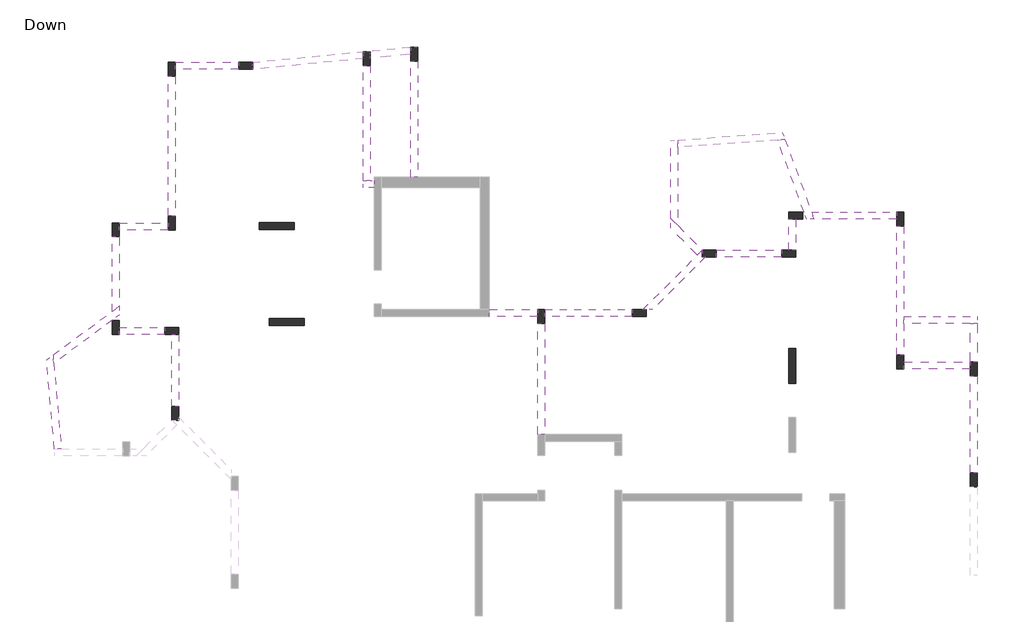
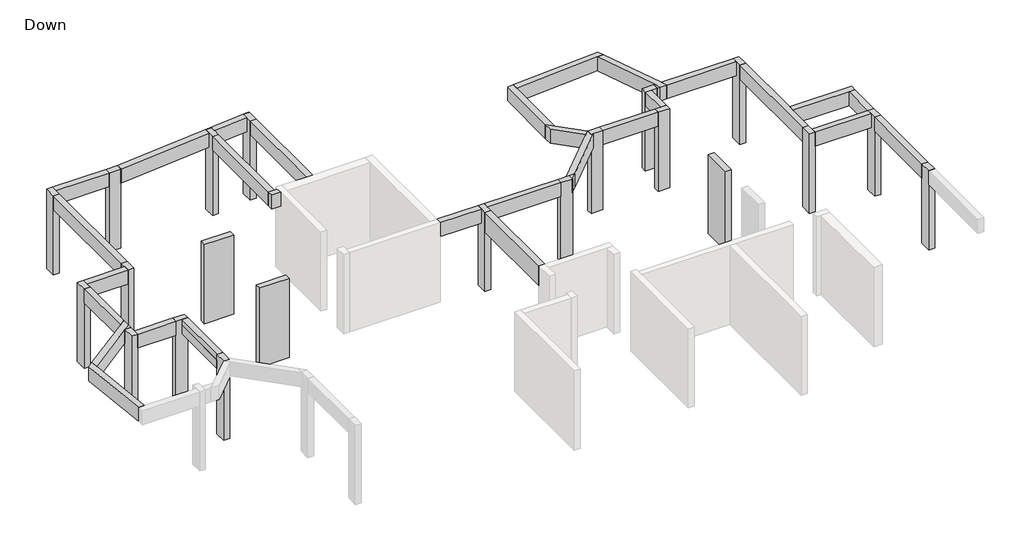
# One storey, part 3 of 3: 28 beams, 21 columns.
"""IFC4 building model written with IfcOpenShell, lengths in millimetres."""

from ifc_helpers import new_model, si_unit, frame, origin, origin_with_axes, place, context, project, spatial, polyline, outline, extrude, faceted_brep, element, save

model = new_model("IFC4")

# Units and contexts
model_context = context("Model", 3, world=origin())
ifc_project = project(units=[si_unit("LENGTHUNIT", "METRE", prefix="MILLI")], contexts=[model_context])

# Site, building, storey
site = spatial("IfcSite", under=ifc_project)
building = spatial("IfcBuilding", under=site)
storey = spatial("IfcBuildingStorey", under=building, Name="Down", Elevation=0.0)

# Beams
placement = place(None, origin())
element("IfcBeam", 1, ObjectType="Concrete Rectengular Beam : 20/50", at=placement, inside=storey, context=model_context, shape_type="Brep", body=[
    faceted_brep([(-18653.293728, -891.3531176, 2850.0), (-18452.5305511, -891.3531176, 2850.0), (-18667.1860705, 1563.4435406, 2850.0), (-18687.6029963, 1796.9311366, 2850.0), (-18876.1976023, 1657.7715773, 2850.0), (-18687.6029963, 1796.9311366, 2350.0), (-18452.5305511, -891.3531176, 2650.0), (-18452.5305511, -891.3531176, 2350.0), (-18667.1860705, 1563.4435406, 2350.0), (-18653.293728, -891.3531176, 2350.0), (-18876.1976023, 1657.7715773, 2350.0)], [[[0, 1, 2, 3, 4]], [[5, 3, 2, 1, 6, 7, 8]], [[7, 9, 10, 5, 8]], [[9, 0, 4, 10]], [[1, 0, 9, 7, 6]], [[4, 3, 5, 10]]]),
])
element("IfcBeam", 2, ObjectType="Concrete Rectengular Beam : 20/50", at=placement, inside=storey, context=model_context, shape_type="Brep", body=[
    faceted_brep([(-18687.6029963, 1796.9311366, 2850.0), (-18667.1860705, 1563.4435406, 2850.0), (-16994.2441564, 2797.8683443, 2850.0), (-16794.2441564, 2945.4436777, 2850.0), (-16794.2441564, 3193.9964468, 2850.0), (-16994.2441564, 3046.4211134, 2850.0), (-16794.2441564, 2945.4436777, 2350.0), (-18667.1860705, 1563.4435406, 2650.0), (-18667.1860705, 1563.4435406, 2350.0), (-16994.2441564, 2797.8683443, 2350.0), (-18687.6029963, 1796.9311366, 2350.0), (-16994.2441564, 3046.4211134, 2350.0), (-16794.2441564, 3193.9964468, 2350.0)], [[[0, 1, 2, 3, 4, 5]], [[6, 3, 2, 1, 7, 8, 9]], [[8, 10, 11, 12, 6, 9]], [[10, 0, 5, 4, 12, 11]], [[1, 0, 10, 8, 7]], [[4, 3, 6, 12]]]),
])
element("IfcBeam", 3, ObjectType="Concrete Rectengular Beam : 20/50", at=placement, inside=storey, context=model_context, shape_type="Brep", body=[
    faceted_brep([(-15089.2187138, 316.4585788, 2850.0), (-15089.2187138, 2386.9126556, 2850.0), (-15284.2187138, 2386.9126556, 2850.0), (-15284.2187138, 316.4585788, 2850.0), (-15089.2187138, 316.4585788, 2650.0), (-15089.2187138, 316.4585788, 2350.0), (-15089.2187138, 2386.9126556, 2350.0), (-15089.2187138, 2386.9126556, 2650.0), (-15289.2187138, 2386.9126556, 2350.0), (-15289.2187138, 316.4585788, 2350.0), (-15289.2187138, 316.4585788, 2650.0), (-15289.2187138, 2386.9126556, 2650.0), (-15284.2187138, 2386.9126556, 2650.0), (-15284.2187138, 316.4585788, 2650.0)], [[[0, 1, 2, 3]], [[1, 0, 4, 5, 6, 7]], [[8, 6, 5, 9]], [[8, 9, 10, 11]], [[6, 8, 11, 12, 2, 1, 7]], [[9, 5, 4, 0, 3, 13, 10]], [[13, 12, 11, 10]], [[12, 13, 3, 2]]]),
])
element("IfcBeam", 4, ObjectType="Concrete Rectengular Beam : 20/50", at=placement, inside=storey, context=model_context, shape_type="Brep", body=[
    faceted_brep([(-16794.2441564, 2586.9126556, 2850.0), (-16794.2441564, 2386.9126556, 2850.0), (-15489.2187138, 2386.9126556, 2850.0), (-15489.2187138, 2586.9126556, 2850.0), (-15489.2187138, 2586.9126556, 2650.0), (-15489.2187138, 2586.9126556, 2350.0), (-16794.2441564, 2586.9126556, 2350.0), (-16794.2441564, 2586.9126556, 2650.0), (-16794.2441564, 2386.9126556, 2350.0), (-15489.2187138, 2386.9126556, 2350.0), (-16794.2441564, 2386.9126556, 2650.0), (-15489.2187138, 2386.9126556, 2650.0)], [[[0, 1, 2, 3]], [[0, 3, 4, 5, 6, 7]], [[8, 6, 5, 9]], [[2, 1, 10, 8, 9, 11]], [[1, 0, 7, 6, 8, 10]], [[3, 2, 11, 9, 5, 4]]]),
])
element("IfcBeam", 5, ObjectType="Concrete Rectengular Beam : 20/50", at=placement, inside=storey, context=model_context, shape_type="Brep", body=[
    faceted_brep([(-16794.2441564, 5184.8420774, 2850.0), (-16994.2441564, 5184.8420774, 2850.0), (-16994.2441564, 3046.4211134, 2850.0), (-16794.2441564, 3193.9964468, 2850.0), (-16794.2441564, 5184.8420774, 2350.0), (-16794.2441564, 3193.9964468, 2350.0), (-16994.2441564, 5184.8420774, 2350.0), (-16994.2441564, 3046.4211134, 2350.0)], [[[0, 1, 2, 3]], [[4, 0, 3, 5]], [[6, 4, 5, 7]], [[1, 6, 7, 2]], [[1, 0, 4, 6]], [[3, 2, 7, 5]]]),
    faceted_brep([(-16794.2441564, 2786.9126556, 2850.0), (-16994.2441564, 2786.9126556, 2850.0), (-16994.2441564, 2786.9126556, 2650.0), (-16994.2441564, 2786.9126556, 2350.0), (-16794.2441564, 2786.9126556, 2350.0), (-16994.2441564, 2797.8683443, 2850.0), (-16794.2441564, 2945.4436777, 2850.0), (-16794.2441564, 2945.4436777, 2350.0), (-16994.2441564, 2797.8683443, 2350.0), (-16994.2441564, 2797.8683443, 2650.0)], [[[0, 1, 2, 3, 4]], [[5, 6, 7, 8, 9]], [[1, 0, 6, 5]], [[0, 4, 7, 6]], [[4, 3, 8, 7]], [[1, 5, 9, 8, 3, 2]]]),
])
element("IfcBeam", 6, ObjectType="Concrete Rectengular Beam : 20/50", at=placement, inside=storey, context=model_context, shape_type="Brep", body=[
    faceted_brep([(-15386.5645409, 5384.8420774, 2850.0), (-15386.5645409, 5584.8420774, 2850.0), (-16794.2441564, 5584.8420774, 2850.0), (-16794.2441564, 5384.8420774, 2850.0), (-15386.5645409, 5584.8420774, 2350.0), (-16794.2441564, 5584.8420774, 2350.0), (-15386.5645409, 5384.8420774, 2350.0), (-16794.2441564, 5384.8420774, 2350.0), (-16794.2441564, 5384.8420774, 2650.0), (-15386.5645409, 5384.8420774, 2650.0)], [[[0, 1, 2, 3]], [[1, 4, 5, 2]], [[4, 6, 7, 5]], [[0, 3, 8, 7, 6, 9]], [[1, 0, 9, 6, 4]], [[3, 2, 5, 7, 8]]]),
])
element("IfcBeam", 7, ObjectType="Concrete Rectengular Beam : 20/50", at=placement, inside=storey, context=model_context, shape_type="Brep", body=[
    faceted_brep([(-15186.5645409, 9788.9617999, 2850.0), (-15386.5645409, 9788.9617999, 2850.0), (-15386.5645409, 5784.8420774, 2850.0), (-15186.5645409, 5784.8420774, 2850.0), (-15186.5645409, 5784.8420774, 2650.0), (-15186.5645409, 5784.8420774, 2350.0), (-15186.5645409, 9788.9617999, 2350.0), (-15186.5645409, 9788.9617999, 2650.0), (-15386.5645409, 9788.9617999, 2350.0), (-15386.5645409, 5784.8420774, 2350.0)], [[[0, 1, 2, 3]], [[0, 3, 4, 5, 6, 7]], [[8, 6, 5, 9]], [[1, 8, 9, 2]], [[1, 0, 7, 6, 8]], [[3, 2, 9, 5, 4]]]),
])
element("IfcBeam", 8, ObjectType="Concrete Rectengular Beam : 20/50", at=placement, inside=storey, context=model_context, shape_type="Brep", body=[
    faceted_brep([(-15186.5645409, 10188.9617999, 2850.0), (-15186.5645409, 9988.9617999, 2850.0), (-13373.5990213, 9988.9617999, 2850.0), (-13373.5990213, 10188.9617999, 2850.0), (-15186.5645409, 9988.9617999, 2650.0), (-15186.5645409, 9988.9617999, 2350.0), (-13373.5990213, 9988.9617999, 2350.0), (-13373.5990213, 9988.9617999, 2650.0), (-15186.5645409, 10188.9617999, 2350.0), (-13373.5990213, 10188.9617999, 2350.0)], [[[0, 1, 2, 3]], [[2, 1, 4, 5, 6, 7]], [[5, 8, 9, 6]], [[8, 0, 3, 9]], [[0, 8, 5, 4, 1]], [[3, 2, 7, 6, 9]]]),
    faceted_brep([(-12973.5990213, 10088.9617999, 2850.0), (-12968.8298625, 9988.9617999, 2850.0), (-12968.8298625, 9988.9617999, 2650.0), (-12968.8298625, 9988.9617999, 2350.0), (-12973.5990213, 10088.9617999, 2350.0), (-12973.5990213, 9988.9617999, 2850.0), (-12973.5990213, 9988.9617999, 2350.0), (-12973.5990213, 9988.9617999, 2650.0)], [[[0, 1, 2, 3, 4]], [[5, 0, 4, 6, 7]], [[1, 0, 5]], [[1, 5, 7, 6, 3, 2]], [[4, 3, 6]]]),
])
element("IfcBeam", 9, ObjectType="Concrete Rectengular Beam : 20/50", at=placement, inside=storey, context=model_context, shape_type="Brep", body=[
    faceted_brep([(-8256.1274624, 10640.4109367, 2850.0), (-12978.3681802, 10188.9617999, 2850.0), (-12973.5990213, 10188.9617999, 2850.0), (-12973.5990213, 10088.9617999, 2850.0), (-12968.8298625, 9988.9617999, 2850.0), (-9797.9493855, 10292.099937, 2850.0), (-9797.9493855, 10422.4041492, 2850.0), (-9797.9493855, 10488.7487212, 2850.0), (-9597.9493855, 10488.7487212, 2850.0), (-9597.9493855, 10422.4041492, 2850.0), (-9597.9493855, 10311.2200609, 2850.0), (-8437.0941181, 10422.1985433, 2850.0), (-8437.0941181, 10622.4041492, 2850.0), (-8254.4060024, 10622.4041492, 2850.0), (-9597.9493855, 10311.2200609, 2650.0), (-9597.9493855, 10311.2200609, 2350.0), (-8437.0941181, 10422.1985433, 2350.0), (-8437.0941181, 10422.1985433, 2650.0), (-12978.3681802, 10188.9617999, 2350.0), (-8256.1274624, 10640.4109367, 2350.0), (-8254.4060024, 10622.4041492, 2350.0), (-8437.0941181, 10622.4041492, 2350.0), (-9597.9493855, 10422.4041492, 2350.0), (-9597.9493855, 10488.7487212, 2350.0), (-9797.9493855, 10488.7487212, 2350.0), (-9797.9493855, 10422.4041492, 2350.0), (-9797.9493855, 10292.099937, 2350.0), (-12968.8298625, 9988.9617999, 2350.0), (-12973.5990213, 10088.9617999, 2350.0), (-12973.5990213, 10188.9617999, 2350.0), (-12968.8298625, 9988.9617999, 2650.0), (-9797.9493855, 10292.099937, 2650.0)], [[[0, 1, 2, 3, 4, 5, 6, 7, 8, 9, 10, 11, 12, 13]], [[11, 10, 14, 15, 16, 17]], [[18, 19, 20, 21, 16, 15, 22, 23, 24, 25, 26, 27, 28, 29]], [[1, 0, 19, 18]], [[4, 3, 28, 27, 30]], [[19, 0, 13, 20]], [[29, 2, 1, 18]], [[2, 29, 28, 3]], [[21, 12, 11, 17, 16]], [[12, 21, 20, 13]], [[24, 7, 6, 5, 31, 26, 25]], [[7, 24, 23, 8]], [[8, 23, 22, 15, 14, 10, 9]], [[5, 4, 30, 27, 26, 31]]]),
])
element("IfcBeam", 10, ObjectType="Concrete Rectengular Beam : 20/50", at=placement, inside=storey, context=model_context, shape_type="Brep", body=[
    faceted_brep([(-8237.0941181, 10222.4041492, 2850.0), (-8437.0941181, 10222.4041492, 2850.0), (-8437.0941181, 6897.8899275, 2850.0), (-8237.0941181, 6897.8899275, 2850.0), (-8437.0941181, 10222.4041492, 2350.0), (-8437.0941181, 6897.8899275, 2350.0), (-8437.0941181, 6897.8899275, 2650.0), (-8237.0941181, 10222.4041492, 2350.0), (-8237.0941181, 6897.8899275, 2350.0)], [[[0, 1, 2, 3]], [[1, 4, 5, 6, 2]], [[4, 7, 8, 5]], [[7, 0, 3, 8]], [[1, 0, 7, 4]], [[3, 2, 6, 5, 8]]]),
])
element("IfcBeam", 11, ObjectType="Concrete Rectengular Beam : 20/50", at=placement, inside=storey, context=model_context, shape_type="Brep", body=[
    faceted_brep([(-9490.6856227, 6598.9542002, 2850.0), (-9490.6856227, 6798.9542002, 2850.0), (-9597.9493855, 6798.9542002, 2850.0), (-9797.9493855, 6798.9542002, 2850.0), (-9797.9493855, 6598.9542002, 2850.0), (-9490.6856227, 6798.9542002, 2650.0), (-9490.6856227, 6798.9542002, 2350.0), (-9597.9493855, 6798.9542002, 2350.0), (-9797.9493855, 6798.9542002, 2350.0), (-9797.9493855, 6798.9542002, 2650.0), (-9490.6856227, 6598.9542002, 2350.0), (-9797.9493855, 6598.9542002, 2350.0), (-9797.9493855, 6598.9542002, 2650.0), (-9490.6856227, 6598.9542002, 2650.0)], [[[0, 1, 2, 3, 4]], [[1, 5, 6, 7, 8, 9, 3, 2]], [[6, 10, 11, 8, 7]], [[0, 4, 12, 11, 10, 13]], [[1, 0, 13, 10, 6, 5]], [[4, 3, 9, 8, 11, 12]]]),
])
element("IfcBeam", 12, ObjectType="Concrete Rectengular Beam : 20/50", at=placement, inside=storey, context=model_context, shape_type="Brep", body=[
    faceted_brep([(-9597.9493855, 10088.7487212, 2850.0), (-9797.9493855, 10088.7487212, 2850.0), (-9797.9493855, 6798.9542002, 2850.0), (-9597.9493855, 6798.9542002, 2850.0), (-9597.9493855, 10088.7487212, 2350.0), (-9597.9493855, 6798.9542002, 2650.0), (-9597.9493855, 6798.9542002, 2350.0), (-9797.9493855, 10088.7487212, 2350.0), (-9797.9493855, 6798.9542002, 2350.0), (-9797.9493855, 10088.7487212, 2650.0), (-9797.9493855, 6798.9542002, 2650.0)], [[[0, 1, 2, 3]], [[4, 0, 3, 5, 6]], [[7, 4, 6, 8]], [[2, 1, 9, 7, 8, 10]], [[1, 0, 4, 7, 9]], [[3, 2, 10, 8, 6, 5]]]),
])
element("IfcBeam", 13, ObjectType="Concrete Rectengular Beam : 20/50", at=placement, inside=storey, context=model_context, shape_type="Brep", body=[
    faceted_brep([(-4797.6379386, 2895.9323955, 2850.0), (-4797.6379386, 3095.9323955, 2850.0), (-6200.1625371, 3095.9323955, 2850.0), (-6200.1625371, 2895.9323955, 2850.0), (-4797.6379386, 3095.9323955, 2350.0), (-6200.1625371, 3095.9323955, 2350.0), (-4797.6379386, 2895.9323955, 2350.0), (-6200.1625371, 2895.9323955, 2350.0), (-6200.1625371, 2895.9323955, 2650.0), (-4797.6379386, 2895.9323955, 2650.0)], [[[0, 1, 2, 3]], [[1, 4, 5, 2]], [[4, 6, 7, 5]], [[0, 3, 8, 7, 6, 9]], [[1, 0, 9, 6, 4]], [[3, 2, 5, 7, 8]]]),
])
element("IfcBeam", 14, ObjectType="Concrete Rectengular Beam : 20/50", at=placement, inside=storey, context=model_context, shape_type="Brep", body=[
    faceted_brep([(-2099.1198792, 2895.9323955, 2850.0), (-2099.1198792, 3095.9323955, 2850.0), (-4597.6379386, 3095.9323955, 2850.0), (-4597.6379386, 2895.9323955, 2850.0), (-4597.6379386, 2895.9323955, 2650.0), (-4597.6379386, 2895.9323955, 2350.0), (-2099.1198792, 2895.9323955, 2350.0), (-2099.1198792, 2895.9323955, 2650.0), (-2099.1198792, 3095.9323955, 2350.0), (-4597.6379386, 3095.9323955, 2350.0)], [[[0, 1, 2, 3]], [[0, 3, 4, 5, 6, 7]], [[8, 6, 5, 9]], [[1, 8, 9, 2]], [[1, 0, 7, 6, 8]], [[3, 2, 9, 5, 4]]]),
    faceted_brep([(-1512.3548664, 3095.9323955, 2850.0), (-1699.1198792, 2909.1673916, 2850.0), (-1699.1198792, 2909.1673916, 2650.0), (-1699.1198792, 2909.1673916, 2350.0), (-1512.3548664, 3095.9323955, 2350.0), (-1512.3548664, 3095.9323955, 2650.0), (-1699.1198792, 3095.9323955, 2850.0), (-1699.1198792, 3095.9323955, 2350.0)], [[[0, 1, 2, 3, 4, 5]], [[1, 6, 7, 3, 2]], [[0, 6, 1]], [[7, 4, 3]], [[6, 0, 5, 4, 7]]]),
])
element("IfcBeam", 15, ObjectType="Concrete Rectengular Beam : 20/50", at=placement, inside=storey, context=model_context, shape_type="Brep", body=[
    faceted_brep([(-9.6892647, 4598.5979252, 2850.0), (-89.77599, 4598.5979252, 2850.0), (-89.77599, 4798.5979252, 2850.0), (-83.949, 4798.5979252, 2850.0), (-88.2404871, 4802.8894122, 2850.0), (-229.6618467, 4661.4680594, 2850.0), (-1795.1975857, 3095.9323955, 2850.0), (-1699.1198792, 3095.9323955, 2850.0), (-1512.3548664, 3095.9323955, 2850.0), (-1512.3548664, 3095.9323955, 2650.0), (-1512.3548664, 3095.9323955, 2350.0), (-9.6892647, 4598.5979252, 2350.0), (-9.6892647, 4598.5979252, 2650.0), (-89.77599, 4598.5979252, 2350.0), (-1699.1198792, 3095.9323955, 2350.0), (-1795.1975857, 3095.9323955, 2350.0), (-229.6618467, 4661.4680594, 2350.0), (-88.2404871, 4802.8894122, 2350.0), (-83.949, 4798.5979252, 2350.0), (-89.77599, 4798.5979252, 2350.0), (-88.2404871, 4802.8894122, 2650.0), (-83.949, 4798.5979252, 2650.0)], [[[0, 1, 2, 3, 4, 5, 6, 7, 8]], [[0, 8, 9, 10, 11, 12]], [[13, 11, 10, 14, 15, 16, 17, 18, 19]], [[15, 6, 5, 4, 20, 17, 16]], [[13, 1, 0, 12, 11]], [[1, 13, 19, 2]], [[8, 7, 6, 15, 14, 10, 9]], [[4, 3, 21, 18, 17, 20]], [[2, 19, 18, 21, 3]]]),
])
element("IfcBeam", 16, ObjectType="Concrete Rectengular Beam : 20/50", at=placement, inside=storey, context=model_context, shape_type="Brep", body=[
    faceted_brep([(-229.6618467, 4661.4680594, 2850.0), (-88.2404871, 4802.8894122, 2850.0), (-799.5327681, 5514.1816932, 2850.0), (-999.5327681, 5714.1816932, 2850.0), (-999.5327681, 5431.3389807, 2850.0), (-999.5327681, 5714.1816932, 2350.0), (-88.2404871, 4802.8894122, 2650.0), (-88.2404871, 4802.8894122, 2350.0), (-799.5327681, 5514.1816932, 2350.0), (-229.6618467, 4661.4680594, 2350.0), (-999.5327681, 5431.3389807, 2350.0)], [[[0, 1, 2, 3, 4]], [[5, 3, 2, 1, 6, 7, 8]], [[7, 9, 10, 5, 8]], [[9, 0, 4, 10]], [[1, 0, 9, 7, 6]], [[4, 3, 5, 10]]]),
])
element("IfcBeam", 17, ObjectType="Concrete Rectengular Beam : 20/50", at=placement, inside=storey, context=model_context, shape_type="Brep", body=[
    faceted_brep([(-999.5327681, 5714.1816932, 2850.0), (-799.5327681, 5514.1816932, 2850.0), (-799.5327681, 7759.5088284, 2850.0), (-799.5327681, 7959.997208, 2850.0), (-999.5327681, 7946.0118456, 2850.0), (-799.5327681, 5514.1816932, 2650.0), (-799.5327681, 5514.1816932, 2350.0), (-799.5327681, 7759.5088284, 2350.0), (-799.5327681, 7959.997208, 2350.0), (-999.5327681, 5714.1816932, 2350.0), (-999.5327681, 7946.0118456, 2350.0)], [[[0, 1, 2, 3, 4]], [[1, 5, 6, 7, 8, 3, 2]], [[6, 9, 10, 8, 7]], [[9, 0, 4, 10]], [[1, 0, 9, 6, 5]], [[4, 3, 8, 10]]]),
])
element("IfcBeam", 18, ObjectType="Concrete Rectengular Beam : 20/50", at=placement, inside=storey, context=model_context, shape_type="Brep", body=[
    faceted_brep([(-799.5327681, 7959.997208, 2850.0), (-799.5327681, 7759.5088284, 2850.0), (2065.6791891, 7959.8639661, 2850.0), (2273.4365693, 7974.3917773, 2850.0), (2201.5390264, 8169.852591, 2850.0), (2273.4365693, 7974.3917773, 2350.0), (-799.5327681, 7759.5088284, 2650.0), (-799.5327681, 7759.5088284, 2350.0), (2065.6791891, 7959.8639661, 2350.0), (-799.5327681, 7959.997208, 2350.0), (2201.5390264, 8169.852591, 2350.0)], [[[0, 1, 2, 3, 4]], [[5, 3, 2, 1, 6, 7, 8]], [[7, 9, 10, 5, 8]], [[9, 0, 4, 10]], [[1, 0, 9, 7, 6]], [[4, 3, 5, 10]]]),
])
element("IfcBeam", 19, ObjectType="Concrete Rectengular Beam : 20/50", at=placement, inside=storey, context=model_context, shape_type="Brep", body=[
    faceted_brep([(2273.4365693, 7974.3917773, 2850.0), (2065.6791891, 7959.8639661, 2850.0), (2826.2618446, 5892.1423364, 2850.0), (2899.8290642, 5692.1423364, 2850.0), (3112.9302979, 5692.1423364, 2850.0), (3039.3630783, 5892.1423364, 2850.0), (2899.8290642, 5692.1423364, 2350.0), (2065.6791891, 7959.8639661, 2650.0), (2065.6791891, 7959.8639661, 2350.0), (2826.2618446, 5892.1423364, 2350.0), (2273.4365693, 7974.3917773, 2350.0), (3039.3630783, 5892.1423364, 2350.0), (3112.9302979, 5692.1423364, 2350.0)], [[[0, 1, 2, 3, 4, 5]], [[6, 3, 2, 1, 7, 8, 9]], [[8, 10, 11, 12, 6, 9]], [[10, 0, 5, 4, 12, 11]], [[1, 0, 10, 8, 7]], [[4, 3, 6, 12]]]),
])
element("IfcBeam", 20, ObjectType="Concrete Rectengular Beam : 20/50", at=placement, inside=storey, context=model_context, shape_type="Brep", body=[
    faceted_brep([(2189.104476, 4598.5979252, 2850.0), (2189.104476, 4798.5979252, 2850.0), (310.22401, 4798.5979252, 2850.0), (310.22401, 4598.5979252, 2850.0), (310.22401, 4598.5979252, 2650.0), (310.22401, 4598.5979252, 2350.0), (2189.104476, 4598.5979252, 2350.0), (2189.104476, 4598.5979252, 2650.0), (2189.104476, 4798.5979252, 2350.0), (310.22401, 4798.5979252, 2350.0)], [[[0, 1, 2, 3]], [[0, 3, 4, 5, 6, 7]], [[8, 6, 5, 9]], [[1, 8, 9, 2]], [[1, 0, 7, 6, 8]], [[3, 2, 9, 5, 4]]]),
])
element("IfcBeam", 21, ObjectType="Concrete Rectengular Beam : 20/50", at=placement, inside=storey, context=model_context, shape_type="Brep", body=[
    faceted_brep([(2589.104476, 5692.1423364, 2850.0), (2389.104476, 5692.1423364, 2850.0), (2389.104476, 4798.5979252, 2850.0), (2589.104476, 4798.5979252, 2850.0), (2389.104476, 5692.1423364, 2650.0), (2389.104476, 5692.1423364, 2350.0), (2389.104476, 4798.5979252, 2350.0), (2389.104476, 4798.5979252, 2650.0), (2589.104476, 5692.1423364, 2350.0), (2589.104476, 4798.5979252, 2350.0), (2589.104476, 4798.5979252, 2650.0), (2589.104476, 5692.1423364, 2650.0)], [[[0, 1, 2, 3]], [[2, 1, 4, 5, 6, 7]], [[5, 8, 9, 6]], [[0, 3, 10, 9, 8, 11]], [[1, 0, 11, 8, 5, 4]], [[3, 2, 7, 6, 9, 10]]]),
])
element("IfcBeam", 22, ObjectType="Concrete Rectengular Beam : 20/50", at=placement, inside=storey, context=model_context, shape_type="Brep", body=[
    faceted_brep([(5484.9828456, 5692.1423364, 2850.0), (5484.9828456, 5892.1423364, 2850.0), (3039.3630783, 5892.1423364, 2850.0), (3112.9302979, 5692.1423364, 2850.0), (5484.9828456, 5692.1423364, 2350.0), (5484.9828456, 5692.1423364, 2650.0), (3112.9302979, 5692.1423364, 2350.0), (5484.9828456, 5892.1423364, 2350.0), (3039.3630783, 5892.1423364, 2350.0)], [[[0, 1, 2, 3]], [[4, 5, 0, 3, 6]], [[7, 4, 6, 8]], [[1, 7, 8, 2]], [[1, 0, 5, 4, 7]], [[3, 2, 8, 6]]]),
    faceted_brep([(2789.104476, 5692.1423364, 2850.0), (2789.104476, 5892.1423364, 2850.0), (2789.104476, 5892.1423364, 2650.0), (2789.104476, 5892.1423364, 2350.0), (2789.104476, 5692.1423364, 2350.0), (2826.2618446, 5892.1423364, 2850.0), (2899.8290642, 5692.1423364, 2850.0), (2899.8290642, 5692.1423364, 2350.0), (2826.2618446, 5892.1423364, 2350.0), (2826.2618446, 5892.1423364, 2650.0)], [[[0, 1, 2, 3, 4]], [[5, 6, 7, 8, 9]], [[1, 0, 6, 5]], [[0, 4, 7, 6]], [[4, 3, 8, 7]], [[1, 5, 9, 8, 3, 2]]]),
])
element("IfcBeam", 23, ObjectType="Concrete Rectengular Beam : 20/50", at=placement, inside=storey, context=model_context, shape_type="Brep", body=[
    faceted_brep([(5484.9828456, 1795.5159248, 2850.0), (5684.9828456, 1795.5159248, 2850.0), (5684.9828456, 2705.1624293, 2850.0), (5684.9828456, 2905.1624293, 2850.0), (5684.9828456, 5494.9383888, 2850.0), (5484.9828456, 5494.9383888, 2850.0), (5484.9828456, 5494.9383888, 2650.0), (5484.9828456, 5494.9383888, 2350.0), (5484.9828456, 1795.5159248, 2350.0), (5484.9828456, 1795.5159248, 2650.0), (5684.9828456, 1795.5159248, 2350.0), (5684.9828456, 5494.9383888, 2350.0), (5684.9828456, 2905.1624293, 2350.0), (5684.9828456, 2705.1624293, 2350.0)], [[[0, 1, 2, 3, 4, 5]], [[0, 5, 6, 7, 8, 9]], [[10, 8, 7, 11, 12, 13]], [[1, 10, 13, 12, 11, 4, 3, 2]], [[1, 0, 9, 8, 10]], [[5, 4, 11, 7, 6]]]),
])
element("IfcBeam", 24, ObjectType="Concrete Rectengular Beam : 20/50", at=placement, inside=storey, context=model_context, shape_type="Brep", body=[
    faceted_brep([(5684.9828456, 2905.1624293, 2850.0), (5684.9828456, 2705.1624293, 2850.0), (7591.3944084, 2705.1624293, 2850.0), (7791.3944084, 2705.1624293, 2850.0), (7791.3944084, 2905.1624293, 2850.0), (5684.9828456, 2705.1624293, 2650.0), (5684.9828456, 2705.1624293, 2350.0), (7591.3944084, 2705.1624293, 2350.0), (7791.3944084, 2705.1624293, 2350.0), (5684.9828456, 2905.1624293, 2350.0), (7791.3944084, 2905.1624293, 2350.0)], [[[0, 1, 2, 3, 4]], [[1, 5, 6, 7, 8, 3, 2]], [[6, 9, 10, 8, 7]], [[9, 0, 4, 10]], [[1, 0, 9, 6, 5]], [[4, 3, 8, 10]]]),
])
element("IfcBeam", 25, ObjectType="Concrete Rectengular Beam : 20/50", at=placement, inside=storey, context=model_context, shape_type="Brep", body=[
    faceted_brep([(7591.3944084, 1595.5159248, 2850.0), (7791.3944084, 1595.5159248, 2850.0), (7791.3944084, 2705.1624293, 2850.0), (7591.3944084, 2705.1624293, 2850.0), (7591.3944084, 1595.5159248, 2350.0), (7591.3944084, 1595.5159248, 2650.0), (7591.3944084, 2705.1624293, 2650.0), (7591.3944084, 2705.1624293, 2350.0), (7791.3944084, 1595.5159248, 2350.0), (7791.3944084, 2705.1624293, 2350.0)], [[[0, 1, 2, 3]], [[4, 5, 0, 3, 6, 7]], [[8, 4, 7, 9]], [[1, 8, 9, 2]], [[1, 0, 5, 4, 8]], [[3, 2, 9, 7, 6]]]),
])
element("IfcBeam", 26, ObjectType="Concrete Rectengular Beam : 20/50", at=placement, inside=storey, context=model_context, shape_type="Brep", body=[
    faceted_brep([(7591.3944084, 1395.5159248, 2850.0), (7591.3944084, 1595.5159248, 2850.0), (5684.9828456, 1595.5159248, 2850.0), (5684.9828456, 1395.5159248, 2850.0), (7591.3944084, 1595.5159248, 2650.0), (7591.3944084, 1595.5159248, 2350.0), (5684.9828456, 1595.5159248, 2350.0), (5684.9828456, 1595.5159248, 2650.0), (7591.3944084, 1395.5159248, 2350.0), (5684.9828456, 1395.5159248, 2350.0), (5684.9828456, 1395.5159248, 2650.0), (7591.3944084, 1395.5159248, 2650.0)], [[[0, 1, 2, 3]], [[1, 4, 5, 6, 7, 2]], [[5, 8, 9, 6]], [[0, 3, 10, 9, 8, 11]], [[1, 0, 11, 8, 5, 4]], [[3, 2, 7, 6, 9, 10]]]),
])
element("IfcBeam", 27, ObjectType="Concrete Rectengular Beam : 20/50", at=placement, inside=storey, context=model_context, shape_type="SweptSolid", body=[
    extrude(outline(polyline([(7791.3944084, -1588.6737606), (7591.3944084, -1588.6737606), (7591.3944084, 1195.5159248), (7791.3944084, 1195.5159248), (7791.3944084, -1588.6737606)])), frame((0.0, 0.0, 2350.0), z_axis=(0.0, 0.0, 1.0), x_axis=(1.0, 0.0, 0.0)), (0.0, 0.0, 1.0), 500.0),
])
element("IfcBeam", 28, ObjectType="Concrete Rectengular Beam : 20/70", at=placement, inside=storey, context=model_context, shape_type="Brep", body=[
    faceted_brep([(-4597.6379386, 2696.2012144, 2850.0), (-4797.6379386, 2696.2012144, 2850.0), (-4797.6379386, -483.2914692, 2850.0), (-4597.6379386, -483.2914692, 2850.0), (-4797.6379386, 2696.2012144, 2650.0), (-4797.6379386, 2696.2012144, 2150.0), (-4797.6379386, -483.2914692, 2150.0), (-4797.6379386, -483.2914692, 2650.0), (-4597.6379386, 2696.2012144, 2150.0), (-4597.6379386, -483.2914692, 2150.0), (-4597.6379386, -483.2914692, 2650.0)], [[[0, 1, 2, 3]], [[2, 1, 4, 5, 6, 7]], [[5, 8, 9, 6]], [[8, 0, 3, 10, 9]], [[1, 0, 8, 5, 4]], [[3, 2, 7, 6, 9, 10]]]),
])

# Columns
element("IfcColumn", 29, ObjectType="Concrete Rectengular Column : 100/20", at=placement, inside=storey, context=model_context, shape_type="Brep", body=[
    faceted_brep([(2387.619868, 1976.5237192, 0.0), (2587.619868, 1976.5237192, 0.0), (2587.619868, 976.5237192, 0.0), (2387.619868, 976.5237192, 0.0), (2387.619868, 1976.5237192, 2850.0), (2587.619868, 1976.5237192, 2850.0), (2587.619868, 1976.5237192, 2650.0), (2387.619868, 1976.5237192, 2650.0), (2587.619868, 976.5237192, 2850.0), (2587.619868, 976.5237192, 2650.0), (2387.619868, 976.5237192, 2850.0), (2387.619868, 976.5237192, 2650.0)], [[[0, 1, 2, 3]], [[4, 5, 6, 1, 0, 7]], [[5, 8, 9, 2, 1, 6]], [[8, 10, 11, 3, 2, 9]], [[10, 4, 7, 0, 3, 11]], [[4, 10, 8, 5]]]),
])
element("IfcColumn", 30, ObjectType="Concrete Rectengular Column : 100/20", at=placement, inside=storey, context=model_context, shape_type="Brep", body=[
    faceted_brep([(-12489.8453542, 2637.5348136, 0.0), (-12489.8453542, 2837.5348136, 0.0), (-11489.8453542, 2837.5348136, 0.0), (-11489.8453542, 2637.5348136, 0.0), (-12489.8453542, 2637.5348136, 2850.0), (-12489.8453542, 2837.5348136, 2850.0), (-12489.8453542, 2837.5348136, 2650.0), (-12489.8453542, 2637.5348136, 2650.0), (-11489.8453542, 2837.5348136, 2850.0), (-11489.8453542, 2837.5348136, 2650.0), (-11489.8453542, 2637.5348136, 2850.0), (-11489.8453542, 2637.5348136, 2650.0)], [[[0, 1, 2, 3]], [[4, 5, 6, 1, 0, 7]], [[5, 8, 9, 2, 1, 6]], [[8, 10, 11, 3, 2, 9]], [[10, 4, 7, 0, 3, 11]], [[4, 10, 8, 5]]]),
])
element("IfcColumn", 31, ObjectType="Concrete Rectengular Column : 100/20", at=placement, inside=storey, context=model_context, shape_type="Brep", body=[
    faceted_brep([(-12783.7609512, 5396.0878026, 0.0), (-12783.7609512, 5596.0878026, 0.0), (-11783.7609512, 5596.0878026, 0.0), (-11783.7609512, 5396.0878026, 0.0), (-12783.7609512, 5396.0878026, 2850.0), (-12783.7609512, 5596.0878026, 2850.0), (-12783.7609512, 5596.0878026, 2650.0), (-12783.7609512, 5396.0878026, 2650.0), (-11783.7609512, 5596.0878026, 2850.0), (-11783.7609512, 5596.0878026, 2650.0), (-11783.7609512, 5396.0878026, 2850.0), (-11783.7609512, 5396.0878026, 2650.0)], [[[0, 1, 2, 3]], [[4, 5, 6, 1, 0, 7]], [[5, 8, 9, 2, 1, 6]], [[8, 10, 11, 3, 2, 9]], [[10, 4, 7, 0, 3, 11]], [[4, 10, 8, 5]]]),
])
element("IfcColumn", 32, ObjectType="Concrete Rectengular Column : 20/40", at=placement, inside=storey, context=model_context, shape_type="Brep", body=[
    faceted_brep([(-15186.5645409, 10188.9617999, 0.0), (-15186.5645409, 9788.9617999, 0.0), (-15386.5645409, 9788.9617999, 0.0), (-15386.5645409, 10188.9617999, 0.0), (-15186.5645409, 10188.9617999, 2850.0), (-15186.5645409, 9988.9617999, 2850.0), (-15186.5645409, 9788.9617999, 2850.0), (-15386.5645409, 9788.9617999, 2850.0), (-15386.5645409, 10188.9617999, 2850.0)], [[[0, 1, 2, 3]], [[4, 5, 6, 1, 0]], [[6, 7, 2, 1]], [[7, 8, 3, 2]], [[8, 4, 0, 3]], [[4, 8, 7, 6, 5]]]),
])
element("IfcColumn", 33, ObjectType="Concrete Rectengular Column : 20/40", at=placement, inside=storey, context=model_context, shape_type="SweptSolid", body=[
    extrude(outline(polyline([(-13373.5990213, 10188.9617999), (-12973.5990213, 10188.9617999), (-12973.5990213, 9988.9617999), (-13373.5990213, 9988.9617999), (-13373.5990213, 10188.9617999)])), origin_with_axes(), (0.0, 0.0, 1.0), 2850.0),
])
element("IfcColumn", 34, ObjectType="Concrete Rectengular Column : 20/40", at=placement, inside=storey, context=model_context, shape_type="Brep", body=[
    faceted_brep([(-9797.9493855, 10088.7487212, 0.0), (-9797.9493855, 10488.7487212, 0.0), (-9597.9493855, 10488.7487212, 0.0), (-9597.9493855, 10088.7487212, 0.0), (-9797.9493855, 10088.7487212, 2850.0), (-9797.9493855, 10292.099937, 2850.0), (-9797.9493855, 10488.7487212, 2850.0), (-9797.9493855, 10488.7487212, 2350.0), (-9597.9493855, 10488.7487212, 2850.0), (-9597.9493855, 10488.7487212, 2350.0), (-9597.9493855, 10311.2200609, 2850.0), (-9597.9493855, 10088.7487212, 2850.0)], [[[0, 1, 2, 3]], [[4, 5, 6, 7, 1, 0]], [[6, 8, 9, 2, 1, 7]], [[8, 10, 11, 3, 2, 9]], [[11, 4, 0, 3]], [[4, 11, 10, 8, 6, 5]]]),
])
element("IfcColumn", 35, ObjectType="Concrete Rectengular Column : 20/40", at=placement, inside=storey, context=model_context, shape_type="Brep", body=[
    faceted_brep([(-8437.0941181, 10222.4041492, 0.0), (-8437.0941181, 10622.4041492, 0.0), (-8237.0941181, 10622.4041492, 0.0), (-8237.0941181, 10222.4041492, 0.0), (-8437.0941181, 10222.4041492, 2850.0), (-8437.0941181, 10422.1985433, 2850.0), (-8437.0941181, 10622.4041492, 2850.0), (-8237.0941181, 10622.4041492, 2850.0), (-8237.0941181, 10222.4041492, 2850.0)], [[[0, 1, 2, 3]], [[4, 5, 6, 1, 0]], [[6, 7, 2, 1]], [[7, 8, 3, 2]], [[8, 4, 0, 3]], [[4, 8, 7, 6, 5]]]),
])
element("IfcColumn", 36, ObjectType="Concrete Rectengular Column : 20/40", at=placement, inside=storey, context=model_context, shape_type="Brep", body=[
    faceted_brep([(-15186.5645409, 5784.8420774, 0.0), (-15186.5645409, 5384.8420774, 0.0), (-15386.5645409, 5384.8420774, 0.0), (-15386.5645409, 5784.8420774, 0.0), (-15186.5645409, 5784.8420774, 2850.0), (-15186.5645409, 5384.8420774, 2850.0), (-15186.5645409, 5384.8420774, 2650.0), (-15386.5645409, 5384.8420774, 2850.0), (-15386.5645409, 5784.8420774, 2850.0)], [[[0, 1, 2, 3]], [[4, 5, 6, 1, 0]], [[5, 7, 2, 1, 6]], [[7, 8, 3, 2]], [[8, 4, 0, 3]], [[4, 8, 7, 5]]]),
])
element("IfcColumn", 37, ObjectType="Concrete Rectengular Column : 20/40", at=placement, inside=storey, context=model_context, shape_type="Brep", body=[
    faceted_brep([(-16794.2441564, 5584.8420774, 0.0), (-16794.2441564, 5184.8420774, 0.0), (-16994.2441564, 5184.8420774, 0.0), (-16994.2441564, 5584.8420774, 0.0), (-16794.2441564, 5584.8420774, 2850.0), (-16794.2441564, 5384.8420774, 2850.0), (-16794.2441564, 5184.8420774, 2850.0), (-16994.2441564, 5184.8420774, 2850.0), (-16994.2441564, 5584.8420774, 2850.0)], [[[0, 1, 2, 3]], [[4, 5, 6, 1, 0]], [[6, 7, 2, 1]], [[7, 8, 3, 2]], [[8, 4, 0, 3]], [[4, 8, 7, 6, 5]]]),
])
element("IfcColumn", 38, ObjectType="Concrete Rectengular Column : 20/40", at=placement, inside=storey, context=model_context, shape_type="Brep", body=[
    faceted_brep([(-16794.2441564, 2786.9126556, 0.0), (-16794.2441564, 2386.9126556, 0.0), (-16994.2441564, 2386.9126556, 0.0), (-16994.2441564, 2786.9126556, 0.0), (-16794.2441564, 2786.9126556, 2850.0), (-16794.2441564, 2586.9126556, 2850.0), (-16794.2441564, 2386.9126556, 2850.0), (-16994.2441564, 2386.9126556, 2850.0), (-16994.2441564, 2386.9126556, 2650.0), (-16994.2441564, 2786.9126556, 2850.0)], [[[0, 1, 2, 3]], [[4, 5, 6, 1, 0]], [[6, 7, 8, 2, 1]], [[7, 9, 3, 2, 8]], [[9, 4, 0, 3]], [[4, 9, 7, 6, 5]]]),
])
element("IfcColumn", 39, ObjectType="Concrete Rectengular Column : 20/40", at=placement, inside=storey, context=model_context, shape_type="Brep", body=[
    faceted_brep([(-15489.2187138, 2586.9126556, 0.0), (-15089.2187138, 2586.9126556, 0.0), (-15089.2187138, 2386.9126556, 0.0), (-15489.2187138, 2386.9126556, 0.0), (-15489.2187138, 2586.9126556, 2850.0), (-15089.2187138, 2586.9126556, 2850.0), (-15089.2187138, 2586.9126556, 2650.0), (-15089.2187138, 2386.9126556, 2850.0), (-15284.2187138, 2386.9126556, 2850.0), (-15489.2187138, 2386.9126556, 2850.0)], [[[0, 1, 2, 3]], [[4, 5, 6, 1, 0]], [[5, 7, 2, 1, 6]], [[7, 8, 9, 3, 2]], [[9, 4, 0, 3]], [[4, 9, 8, 7, 5]]]),
])
element("IfcColumn", 40, ObjectType="Concrete Rectengular Column : 20/40", at=placement, inside=storey, context=model_context, shape_type="Brep", body=[
    faceted_brep([(-15289.2187138, -83.5414212, 0.0), (-15289.2187138, 316.4585788, 0.0), (-15089.2187138, 316.4585788, 0.0), (-15089.2187138, -83.5414212, 0.0), (-15289.2187138, -83.5414212, 2850.0), (-15289.2187138, -73.3367957, 2850.0), (-15289.2187138, 316.4585788, 2850.0), (-15289.2187138, 316.4585788, 2650.0), (-15289.2187138, -83.5414212, 2350.0), (-15284.2187138, 316.4585788, 2850.0), (-15089.2187138, 316.4585788, 2850.0), (-15089.2187138, 11.75673, 2850.0), (-15089.2187138, -83.5414212, 2850.0), (-15273.253528, -83.5414212, 2850.0)], [[[0, 1, 2, 3]], [[4, 5, 6, 7, 1, 0, 8]], [[6, 9, 10, 2, 1, 7]], [[10, 11, 12, 3, 2]], [[12, 13, 4, 8, 0, 3]], [[4, 13, 12, 11, 10, 9, 6, 5]]]),
])
element("IfcColumn", 41, ObjectType="Concrete Rectengular Column : 20/40", at=placement, inside=storey, context=model_context, shape_type="SweptSolid", body=[
    extrude(outline(polyline([(7791.3944084, -1588.6737606), (7791.3944084, -1988.6737606), (7591.3944084, -1988.6737606), (7591.3944084, -1588.6737606), (7791.3944084, -1588.6737606)])), origin_with_axes(), (0.0, 0.0, 1.0), 2850.0),
])
element("IfcColumn", 42, ObjectType="Concrete Rectengular Column : 20/40", at=placement, inside=storey, context=model_context, shape_type="Brep", body=[
    faceted_brep([(7591.3944084, 1195.5159248, 0.0), (7591.3944084, 1595.5159248, 0.0), (7791.3944084, 1595.5159248, 0.0), (7791.3944084, 1195.5159248, 0.0), (7591.3944084, 1195.5159248, 2850.0), (7591.3944084, 1395.5159248, 2850.0), (7591.3944084, 1595.5159248, 2850.0), (7791.3944084, 1595.5159248, 2850.0), (7791.3944084, 1195.5159248, 2850.0)], [[[0, 1, 2, 3]], [[4, 5, 6, 1, 0]], [[6, 7, 2, 1]], [[7, 8, 3, 2]], [[8, 4, 0, 3]], [[4, 8, 7, 6, 5]]]),
])
element("IfcColumn", 43, ObjectType="Concrete Rectengular Column : 20/40", at=placement, inside=storey, context=model_context, shape_type="Brep", body=[
    faceted_brep([(5484.9828456, 1395.5159248, 0.0), (5484.9828456, 1795.5159248, 0.0), (5684.9828456, 1795.5159248, 0.0), (5684.9828456, 1395.5159248, 0.0), (5484.9828456, 1395.5159248, 2850.0), (5484.9828456, 1795.5159248, 2850.0), (5484.9828456, 1395.5159248, 2650.0), (5684.9828456, 1795.5159248, 2850.0), (5684.9828456, 1595.5159248, 2850.0), (5684.9828456, 1395.5159248, 2850.0)], [[[0, 1, 2, 3]], [[4, 5, 1, 0, 6]], [[5, 7, 2, 1]], [[7, 8, 9, 3, 2]], [[9, 4, 6, 0, 3]], [[4, 9, 8, 7, 5]]]),
])
element("IfcColumn", 44, ObjectType="Concrete Rectengular Column : 20/40", at=placement, inside=storey, context=model_context, shape_type="Brep", body=[
    faceted_brep([(5484.9828456, 5494.9383888, 0.0), (5484.9828456, 5894.9383888, 0.0), (5684.9828456, 5894.9383888, 0.0), (5684.9828456, 5494.9383888, 0.0), (5484.9828456, 5494.9383888, 2850.0), (5484.9828456, 5692.1423364, 2850.0), (5484.9828456, 5894.9383888, 2850.0), (5684.9828456, 5894.9383888, 2850.0), (5684.9828456, 5494.9383888, 2850.0)], [[[0, 1, 2, 3]], [[4, 5, 6, 1, 0]], [[6, 7, 2, 1]], [[7, 8, 3, 2]], [[8, 4, 0, 3]], [[4, 8, 7, 6, 5]]]),
])
element("IfcColumn", 45, ObjectType="Concrete Rectengular Column : 20/40", at=placement, inside=storey, context=model_context, shape_type="Brep", body=[
    faceted_brep([(2789.104476, 5692.1423364, 0.0), (2389.104476, 5692.1423364, 0.0), (2389.104476, 5892.1423364, 0.0), (2789.104476, 5892.1423364, 0.0), (2789.104476, 5692.1423364, 2850.0), (2589.104476, 5692.1423364, 2850.0), (2389.104476, 5692.1423364, 2850.0), (2389.104476, 5892.1423364, 2850.0), (2389.104476, 5892.1423364, 2650.0), (2789.104476, 5892.1423364, 2850.0)], [[[0, 1, 2, 3]], [[4, 5, 6, 1, 0]], [[6, 7, 8, 2, 1]], [[7, 9, 3, 2, 8]], [[9, 4, 0, 3]], [[4, 9, 7, 6, 5]]]),
])
element("IfcColumn", 46, ObjectType="Concrete Rectengular Column : 20/40", at=placement, inside=storey, context=model_context, shape_type="Brep", body=[
    faceted_brep([(2589.104476, 4598.5979252, 0.0), (2189.104476, 4598.5979252, 0.0), (2189.104476, 4798.5979252, 0.0), (2589.104476, 4798.5979252, 0.0), (2589.104476, 4598.5979252, 2850.0), (2189.104476, 4598.5979252, 2850.0), (2589.104476, 4598.5979252, 2650.0), (2189.104476, 4798.5979252, 2850.0), (2389.104476, 4798.5979252, 2850.0), (2589.104476, 4798.5979252, 2850.0)], [[[0, 1, 2, 3]], [[4, 5, 1, 0, 6]], [[5, 7, 2, 1]], [[7, 8, 9, 3, 2]], [[9, 4, 6, 0, 3]], [[4, 9, 8, 7, 5]]]),
])
element("IfcColumn", 47, ObjectType="Concrete Rectengular Column : 20/40", at=placement, inside=storey, context=model_context, shape_type="Brep", body=[
    faceted_brep([(310.22401, 4598.5979252, 0.0), (-89.77599, 4598.5979252, 0.0), (-89.77599, 4798.5979252, 0.0), (310.22401, 4798.5979252, 0.0), (310.22401, 4598.5979252, 2850.0), (-9.6893457, 4598.5979252, 2850.0), (-89.77599, 4598.5979252, 2850.0), (-89.77599, 4798.5979252, 2850.0), (-83.949, 4798.5979252, 2850.0), (310.22401, 4798.5979252, 2850.0)], [[[0, 1, 2, 3]], [[4, 5, 6, 1, 0]], [[6, 7, 2, 1]], [[7, 8, 9, 3, 2]], [[9, 4, 0, 3]], [[4, 9, 8, 7, 6, 5]]]),
])
element("IfcColumn", 48, ObjectType="Concrete Rectengular Column : 20/40", at=placement, inside=storey, context=model_context, shape_type="Brep", body=[
    faceted_brep([(-1699.1198792, 2895.9323955, 0.0), (-2099.1198792, 2895.9323955, 0.0), (-2099.1198792, 3095.9323955, 0.0), (-1699.1198792, 3095.9323955, 0.0), (-1699.1198792, 2895.9323955, 2850.0), (-2099.1198792, 2895.9323955, 2850.0), (-1699.1198792, 2895.9323955, 2650.0), (-2099.1198792, 3095.9323955, 2850.0), (-1699.1198792, 3095.9323955, 2850.0), (-1699.1198792, 2909.1673916, 2850.0)], [[[0, 1, 2, 3]], [[4, 5, 1, 0, 6]], [[5, 7, 2, 1]], [[7, 8, 3, 2]], [[8, 9, 4, 6, 0, 3]], [[4, 9, 8, 7, 5]]]),
])
element("IfcColumn", 49, ObjectType="Concrete Rectengular Column : 20/40", at=placement, inside=storey, context=model_context, shape_type="Brep", body=[
    faceted_brep([(-4597.6379386, 3096.2012144, 0.0), (-4597.6379386, 2696.2012144, 0.0), (-4797.6379386, 2696.2012144, 0.0), (-4797.6379386, 3096.2012144, 0.0), (-4597.6379386, 3096.2012144, 2850.0), (-4597.6379386, 2895.9323955, 2850.0), (-4597.6379386, 2696.2012144, 2850.0), (-4797.6379386, 2696.2012144, 2850.0), (-4797.6379386, 2895.9323955, 2850.0), (-4797.6379386, 3096.2012144, 2850.0)], [[[0, 1, 2, 3]], [[4, 5, 6, 1, 0]], [[6, 7, 2, 1]], [[7, 8, 9, 3, 2]], [[9, 4, 0, 3]], [[4, 9, 8, 7, 6, 5]]]),
])

save(model, "model.ifc")

# Revit data of these elements
# Type "Concrete Rectengular Beam : 20/50"
#   Length [instance default] = 152.4 cm
#   b = 20 cm
#   h = 50 cm
#   Structural Material [instance default] = Concrete
#   Assembly Code = ""
# Type "Concrete Rectengular Beam : 20/70"
#   Length [instance default] = 152.4 cm
#   b = 20 cm
#   h = 70 cm
#   Structural Material [instance default] = Concrete
#   Assembly Code = ""
# Type "Concrete Rectengular Column : 100/20"
#   b = 100 cm
#   h = 20 cm
#   Structural Material [instance default] = Concrete
# Type "Concrete Rectengular Column : 20/40"
#   b = 20 cm
#   h = 40 cm
#   Structural Material [instance default] = Concrete
# Element 1 (IfcBeam, "Concrete Rectengular Beam : 20/50")
#   Comments = ""
#   Mark = "B22"
#   SOFiSTiK_AMG_Comments = ""
#   SOFiSTiK_AMG_Scheduled = yes
#   SOFiSTiK_AMG_Adjusted = yes
#   Structural Material = Concrete
#   Phase Created = New Construction
#   Materials on its faces: "Concrete"
# Element 2 (IfcBeam, "Concrete Rectengular Beam : 20/50")
#   Comments = ""
#   Mark = "B23"
#   SOFiSTiK_AMG_Comments = ""
#   SOFiSTiK_AMG_Scheduled = yes
#   SOFiSTiK_AMG_Adjusted = yes
#   Structural Material = Concrete
#   Phase Created = New Construction
#   Materials on its faces: "Concrete"
# Element 3 (IfcBeam, "Concrete Rectengular Beam : 20/50")
#   Comments = ""
#   Mark = "B24"
#   SOFiSTiK_AMG_Comments = ""
#   SOFiSTiK_AMG_Scheduled = yes
#   SOFiSTiK_AMG_Adjusted = yes
#   Structural Material = Concrete
#   Phase Created = New Construction
#   Materials on its faces: "Concrete"
# Element 4 (IfcBeam, "Concrete Rectengular Beam : 20/50")
#   Comments = ""
#   Mark = "B25"
#   SOFiSTiK_AMG_Comments = ""
#   SOFiSTiK_AMG_Scheduled = yes
#   SOFiSTiK_AMG_Adjusted = yes
#   Structural Material = Concrete
#   Phase Created = New Construction
#   Materials on its faces: "Concrete"
# Element 5 (IfcBeam, "Concrete Rectengular Beam : 20/50")
#   Comments = ""
#   Mark = "B26"
#   SOFiSTiK_AMG_Comments = ""
#   SOFiSTiK_AMG_Scheduled = yes
#   SOFiSTiK_AMG_Adjusted = yes
#   Structural Material = Concrete
#   Phase Created = New Construction
#   Materials on its faces: "Concrete"
# Element 6 (IfcBeam, "Concrete Rectengular Beam : 20/50")
#   Comments = ""
#   Mark = "B27"
#   SOFiSTiK_AMG_Comments = ""
#   SOFiSTiK_AMG_Scheduled = yes
#   SOFiSTiK_AMG_Adjusted = yes
#   Structural Material = Concrete
#   Phase Created = New Construction
#   Materials on its faces: "Concrete"
# Element 7 (IfcBeam, "Concrete Rectengular Beam : 20/50")
#   Comments = ""
#   Mark = "B28"
#   SOFiSTiK_AMG_Comments = ""
#   SOFiSTiK_AMG_Scheduled = yes
#   SOFiSTiK_AMG_Adjusted = yes
#   Structural Material = Concrete
#   Phase Created = New Construction
#   Materials on its faces: "Concrete"
# Element 8 (IfcBeam, "Concrete Rectengular Beam : 20/50")
#   Comments = ""
#   Mark = "B30"
#   SOFiSTiK_AMG_Comments = ""
#   SOFiSTiK_AMG_Scheduled = yes
#   SOFiSTiK_AMG_Adjusted = yes
#   Structural Material = Concrete
#   Phase Created = New Construction
#   Materials on its faces: "Concrete"
# Element 9 (IfcBeam, "Concrete Rectengular Beam : 20/50")
#   Comments = ""
#   Mark = "B32"
#   SOFiSTiK_AMG_Comments = ""
#   SOFiSTiK_AMG_Scheduled = yes
#   SOFiSTiK_AMG_Adjusted = yes
#   Structural Material = Concrete
#   Phase Created = New Construction
#   Materials on its faces: "Concrete"
# Element 10 (IfcBeam, "Concrete Rectengular Beam : 20/50")
#   Comments = ""
#   Mark = "B33"
#   SOFiSTiK_AMG_Comments = ""
#   SOFiSTiK_AMG_Scheduled = yes
#   SOFiSTiK_AMG_Adjusted = yes
#   Structural Material = Concrete
#   Phase Created = New Construction
#   Materials on its faces: "Concrete"
# Element 11 (IfcBeam, "Concrete Rectengular Beam : 20/50")
#   Comments = ""
#   Mark = "B34"
#   SOFiSTiK_AMG_Comments = ""
#   SOFiSTiK_AMG_Scheduled = yes
#   SOFiSTiK_AMG_Adjusted = yes
#   Structural Material = Concrete
#   Phase Created = New Construction
#   Materials on its faces: "Concrete"
# Element 12 (IfcBeam, "Concrete Rectengular Beam : 20/50")
#   Comments = ""
#   Mark = "B35"
#   SOFiSTiK_AMG_Comments = ""
#   SOFiSTiK_AMG_Scheduled = yes
#   SOFiSTiK_AMG_Adjusted = yes
#   Structural Material = Concrete
#   Phase Created = New Construction
#   Materials on its faces: "Concrete"
# Element 13 (IfcBeam, "Concrete Rectengular Beam : 20/50")
#   Comments = ""
#   Mark = "B36"
#   SOFiSTiK_AMG_Comments = ""
#   SOFiSTiK_AMG_Scheduled = yes
#   SOFiSTiK_AMG_Adjusted = yes
#   Structural Material = Concrete
#   Phase Created = New Construction
#   Materials on its faces: "Concrete"
# Element 14 (IfcBeam, "Concrete Rectengular Beam : 20/50")
#   Comments = ""
#   Mark = "B37"
#   SOFiSTiK_AMG_Comments = ""
#   SOFiSTiK_AMG_Scheduled = yes
#   SOFiSTiK_AMG_Adjusted = yes
#   Structural Material = Concrete
#   Phase Created = New Construction
#   Materials on its faces: "Concrete"
# Element 15 (IfcBeam, "Concrete Rectengular Beam : 20/50")
#   Comments = ""
#   Mark = "B38"
#   SOFiSTiK_AMG_Comments = ""
#   SOFiSTiK_AMG_Scheduled = yes
#   SOFiSTiK_AMG_Adjusted = yes
#   Structural Material = Concrete
#   Phase Created = New Construction
#   Materials on its faces: "Concrete"
# Element 16 (IfcBeam, "Concrete Rectengular Beam : 20/50")
#   Comments = ""
#   Mark = "B39"
#   SOFiSTiK_AMG_Comments = ""
#   SOFiSTiK_AMG_Scheduled = yes
#   SOFiSTiK_AMG_Adjusted = yes
#   Structural Material = Concrete
#   Phase Created = New Construction
#   Materials on its faces: "Concrete"
# Element 17 (IfcBeam, "Concrete Rectengular Beam : 20/50")
#   Comments = ""
#   Mark = "B40"
#   SOFiSTiK_AMG_Comments = ""
#   SOFiSTiK_AMG_Scheduled = yes
#   SOFiSTiK_AMG_Adjusted = yes
#   Structural Material = Concrete
#   Phase Created = New Construction
#   Materials on its faces: "Concrete"
# Element 18 (IfcBeam, "Concrete Rectengular Beam : 20/50")
#   Comments = ""
#   Mark = "B41"
#   SOFiSTiK_AMG_Comments = ""
#   SOFiSTiK_AMG_Scheduled = yes
#   SOFiSTiK_AMG_Adjusted = yes
#   Structural Material = Concrete
#   Phase Created = New Construction
#   Materials on its faces: "Concrete"
# Element 19 (IfcBeam, "Concrete Rectengular Beam : 20/50")
#   Comments = ""
#   Mark = "B42"
#   SOFiSTiK_AMG_Comments = ""
#   SOFiSTiK_AMG_Scheduled = yes
#   SOFiSTiK_AMG_Adjusted = yes
#   Structural Material = Concrete
#   Phase Created = New Construction
#   Materials on its faces: "Concrete"
# Element 20 (IfcBeam, "Concrete Rectengular Beam : 20/50")
#   Comments = ""
#   Mark = "B43"
#   SOFiSTiK_AMG_Comments = ""
#   SOFiSTiK_AMG_Scheduled = yes
#   SOFiSTiK_AMG_Adjusted = yes
#   Structural Material = Concrete
#   Phase Created = New Construction
#   Materials on its faces: "Concrete"
# Element 21 (IfcBeam, "Concrete Rectengular Beam : 20/50")
#   Comments = ""
#   Mark = "B44"
#   SOFiSTiK_AMG_Comments = ""
#   SOFiSTiK_AMG_Scheduled = yes
#   SOFiSTiK_AMG_Adjusted = yes
#   Structural Material = Concrete
#   Phase Created = New Construction
#   Materials on its faces: "Concrete"
# Element 22 (IfcBeam, "Concrete Rectengular Beam : 20/50")
#   Comments = ""
#   Mark = "B45"
#   SOFiSTiK_AMG_Comments = ""
#   SOFiSTiK_AMG_Scheduled = yes
#   SOFiSTiK_AMG_Adjusted = yes
#   Structural Material = Concrete
#   Phase Created = New Construction
#   Materials on its faces: "Concrete"
# Element 23 (IfcBeam, "Concrete Rectengular Beam : 20/50")
#   Comments = ""
#   Mark = "B46"
#   SOFiSTiK_AMG_Comments = ""
#   SOFiSTiK_AMG_Scheduled = yes
#   SOFiSTiK_AMG_Adjusted = yes
#   Structural Material = Concrete
#   Phase Created = New Construction
#   Materials on its faces: "Concrete"
# Element 24 (IfcBeam, "Concrete Rectengular Beam : 20/50")
#   Comments = ""
#   Mark = "B47"
#   SOFiSTiK_AMG_Comments = ""
#   SOFiSTiK_AMG_Scheduled = yes
#   SOFiSTiK_AMG_Adjusted = yes
#   Structural Material = Concrete
#   Phase Created = New Construction
#   Materials on its faces: "Concrete"
# Element 25 (IfcBeam, "Concrete Rectengular Beam : 20/50")
#   Comments = ""
#   Mark = "B48"
#   SOFiSTiK_AMG_Comments = ""
#   SOFiSTiK_AMG_Scheduled = yes
#   SOFiSTiK_AMG_Adjusted = yes
#   Structural Material = Concrete
#   Phase Created = New Construction
#   Materials on its faces: "Concrete"
# Element 26 (IfcBeam, "Concrete Rectengular Beam : 20/50")
#   Comments = ""
#   Mark = "B49"
#   SOFiSTiK_AMG_Comments = ""
#   SOFiSTiK_AMG_Scheduled = yes
#   SOFiSTiK_AMG_Adjusted = yes
#   Structural Material = Concrete
#   Phase Created = New Construction
#   Materials on its faces: "Concrete"
# Element 27 (IfcBeam, "Concrete Rectengular Beam : 20/50")
#   Comments = ""
#   Mark = "B50"
#   SOFiSTiK_AMG_Comments = ""
#   SOFiSTiK_AMG_Scheduled = yes
#   SOFiSTiK_AMG_Adjusted = yes
#   Structural Material = Concrete
#   Phase Created = New Construction
#   Materials on its faces: "Concrete"
# Element 28 (IfcBeam, "Concrete Rectengular Beam : 20/70")
#   Comments = ""
#   Mark = "B69"
#   SOFiSTiK_AMG_Comments = ""
#   SOFiSTiK_AMG_Scheduled = yes
#   SOFiSTiK_AMG_Adjusted = yes
#   Structural Material = Concrete
#   Phase Created = New Construction
#   Materials on its faces: "Concrete"
# Element 29 (IfcColumn, "Concrete Rectengular Column : 100/20")
#   Comments = ""
#   Mark = "C4"
#   SOFiSTiK_AMG_Comments = ""
#   SOFiSTiK_AMG_Scheduled = yes
#   SOFiSTiK_AMG_Adjusted = yes
#   Structural Material = Concrete
#   Phase Created = New Construction
#   Materials on its faces: "Concrete"
# Element 30 (IfcColumn, "Concrete Rectengular Column : 100/20")
#   Comments = ""
#   Mark = "C5"
#   SOFiSTiK_AMG_Comments = ""
#   SOFiSTiK_AMG_Scheduled = yes
#   SOFiSTiK_AMG_Adjusted = yes
#   Structural Material = Concrete
#   Phase Created = New Construction
#   Materials on its faces: "Concrete"
# Element 31 (IfcColumn, "Concrete Rectengular Column : 100/20")
#   Comments = ""
#   Mark = "C6"
#   SOFiSTiK_AMG_Comments = ""
#   SOFiSTiK_AMG_Scheduled = yes
#   SOFiSTiK_AMG_Adjusted = yes
#   Structural Material = Concrete
#   Phase Created = New Construction
#   Materials on its faces: "Concrete"
# Element 32 (IfcColumn, "Concrete Rectengular Column : 20/40")
#   Comments = ""
#   Mark = "C7"
#   SOFiSTiK_AMG_Comments = ""
#   SOFiSTiK_AMG_Scheduled = yes
#   SOFiSTiK_AMG_Adjusted = yes
#   Structural Material = Concrete
#   Phase Created = New Construction
#   Materials on its faces: "Concrete"
# Element 33 (IfcColumn, "Concrete Rectengular Column : 20/40")
#   Comments = ""
#   Mark = "C8"
#   SOFiSTiK_AMG_Comments = ""
#   SOFiSTiK_AMG_Scheduled = yes
#   SOFiSTiK_AMG_Adjusted = yes
#   Structural Material = Concrete
#   Phase Created = New Construction
#   Materials on its faces: "Concrete"
# Element 34 (IfcColumn, "Concrete Rectengular Column : 20/40")
#   Comments = ""
#   Mark = "C9"
#   SOFiSTiK_AMG_Comments = ""
#   SOFiSTiK_AMG_Scheduled = yes
#   SOFiSTiK_AMG_Adjusted = yes
#   Structural Material = Concrete
#   Phase Created = New Construction
#   Materials on its faces: "Concrete"
# Element 35 (IfcColumn, "Concrete Rectengular Column : 20/40")
#   Comments = ""
#   Mark = "C10"
#   SOFiSTiK_AMG_Comments = ""
#   SOFiSTiK_AMG_Scheduled = yes
#   SOFiSTiK_AMG_Adjusted = yes
#   Structural Material = Concrete
#   Phase Created = New Construction
#   Materials on its faces: "Concrete"
# Element 36 (IfcColumn, "Concrete Rectengular Column : 20/40")
#   Comments = ""
#   Mark = "C11"
#   SOFiSTiK_AMG_Comments = ""
#   SOFiSTiK_AMG_Scheduled = yes
#   SOFiSTiK_AMG_Adjusted = yes
#   Structural Material = Concrete
#   Phase Created = New Construction
#   Materials on its faces: "Concrete"
# Element 37 (IfcColumn, "Concrete Rectengular Column : 20/40")
#   Comments = ""
#   Mark = "C12"
#   SOFiSTiK_AMG_Comments = ""
#   SOFiSTiK_AMG_Scheduled = yes
#   SOFiSTiK_AMG_Adjusted = yes
#   Structural Material = Concrete
#   Phase Created = New Construction
#   Materials on its faces: "Concrete"
# Element 38 (IfcColumn, "Concrete Rectengular Column : 20/40")
#   Comments = ""
#   Mark = "C13"
#   SOFiSTiK_AMG_Comments = ""
#   SOFiSTiK_AMG_Scheduled = yes
#   SOFiSTiK_AMG_Adjusted = yes
#   Structural Material = Concrete
#   Phase Created = New Construction
#   Materials on its faces: "Concrete"
# Element 39 (IfcColumn, "Concrete Rectengular Column : 20/40")
#   Comments = ""
#   Mark = "C14"
#   SOFiSTiK_AMG_Comments = ""
#   SOFiSTiK_AMG_Scheduled = yes
#   SOFiSTiK_AMG_Adjusted = yes
#   Structural Material = Concrete
#   Phase Created = New Construction
#   Materials on its faces: "Concrete"
# Element 40 (IfcColumn, "Concrete Rectengular Column : 20/40")
#   Comments = ""
#   Mark = "C15"
#   SOFiSTiK_AMG_Comments = ""
#   SOFiSTiK_AMG_Scheduled = yes
#   SOFiSTiK_AMG_Adjusted = yes
#   Structural Material = Concrete
#   Phase Created = New Construction
#   Materials on its faces: "Concrete"
# Element 41 (IfcColumn, "Concrete Rectengular Column : 20/40")
#   Comments = ""
#   Mark = "C38"
#   SOFiSTiK_AMG_Comments = ""
#   SOFiSTiK_AMG_Scheduled = yes
#   SOFiSTiK_AMG_Adjusted = yes
#   Structural Material = Concrete
#   Phase Created = New Construction
#   Materials on its faces: "Concrete"
# Element 42 (IfcColumn, "Concrete Rectengular Column : 20/40")
#   Comments = ""
#   Mark = "C40"
#   SOFiSTiK_AMG_Comments = ""
#   SOFiSTiK_AMG_Scheduled = yes
#   SOFiSTiK_AMG_Adjusted = yes
#   Structural Material = Concrete
#   Phase Created = New Construction
#   Materials on its faces: "Concrete"
# Element 43 (IfcColumn, "Concrete Rectengular Column : 20/40")
#   Comments = ""
#   Mark = "C41"
#   SOFiSTiK_AMG_Comments = ""
#   SOFiSTiK_AMG_Scheduled = yes
#   SOFiSTiK_AMG_Adjusted = yes
#   Structural Material = Concrete
#   Phase Created = New Construction
